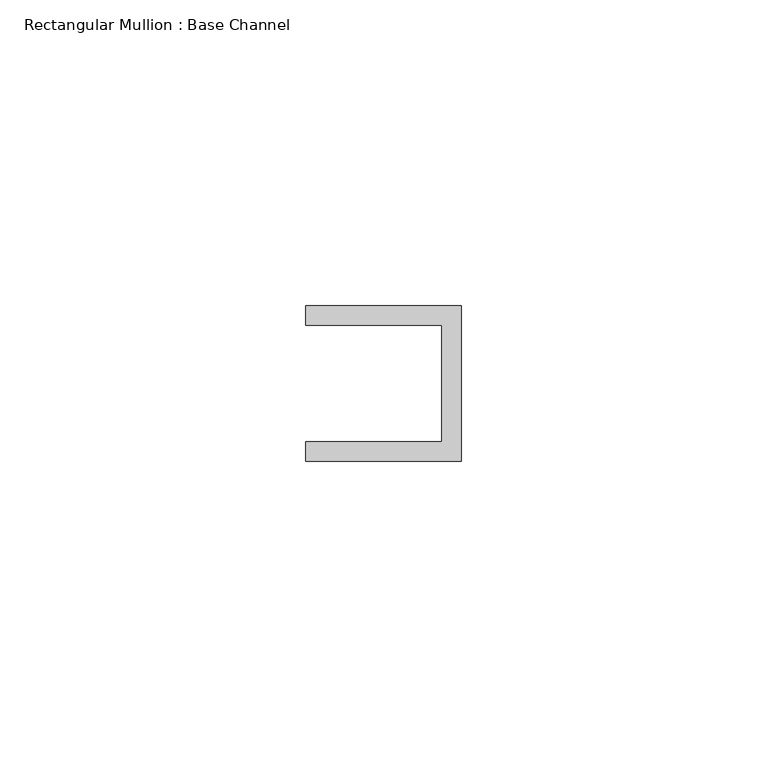
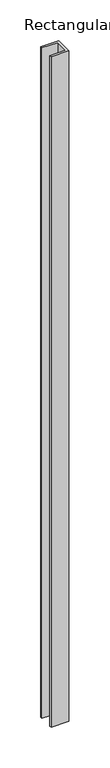
"""IFC4 building model written with IfcOpenShell, lengths in millimetres: member geometry, Rectangular Mullion : Base Channel."""

import ifcopenshell
import ifcopenshell.guid

model = None  # the IFC model being written
_history = None  # IfcOwnerHistory: only IFC2X3 demands one
_inside = {}  # id of a spatial element -> (the spatial element, [elements in it])
_under = {}  # id of a project, library or spatial element -> (it, [spatial elements below it])
_declared = {}  # id of a project -> (the project, [libraries it declares])
_typed = {}  # id of a type object -> (the type object, [elements of that type])
_made_of = {}  # id of a material, layer set ... -> (it, [elements and type objects made of it])


def new_model(schema):
    """Start an empty IFC model of exactly this schema.

    Asked for "IFC4X3", IfcOpenShell would pick the latest addendum, in which some entities
    have other attributes; the version numbers below select the first issue.
    IFC2X3 requires an IfcOwnerHistory on every rooted entity: one is made here for all.
    """
    global model, _history
    if schema == "IFC4X3":
        model = ifcopenshell.file(schema_version=(4, 3, 0, 0))
    else:
        model = ifcopenshell.file(schema=schema)
    _inside.clear()
    _under.clear()
    _declared.clear()
    _typed.clear()
    _made_of.clear()
    _history = None
    if model.schema == "IFC2X3":
        org = make("IfcOrganization", Name="unknown")
        user = make(
            "IfcPersonAndOrganization",
            ThePerson=make("IfcPerson", FamilyName="unknown"),
            TheOrganization=org,
        )
        app = make(
            "IfcApplication",
            ApplicationDeveloper=org,
            Version="unknown",
            ApplicationFullName="unknown",
            ApplicationIdentifier="unknown",
        )
        _history = make(
            "IfcOwnerHistory",
            OwningUser=user,
            OwningApplication=app,
            ChangeAction="ADDED",
            CreationDate=0,
        )
    return model


def make(cls, **values):
    """One entity of the class cls with the attributes given. An attribute that is None is left unset."""
    return model.create_entity(
        cls, **{name: value for name, value in values.items() if value is not None}
    )


def rooted(cls, **values):
    """An entity with a GlobalId (a new one), such as an element, a storey or a relation."""
    return make(cls, GlobalId=ifcopenshell.guid.new(), OwnerHistory=_history, **values)


def si_unit(unit_type, name, prefix=None):
    """IfcSIUnit, for example si_unit("LENGTHUNIT", "METRE", prefix="MILLI")."""
    return make("IfcSIUnit", UnitType=unit_type, Prefix=prefix, Name=name)


def assignment(units):
    """IfcUnitAssignment: the units of a project."""
    return None if units is None else make("IfcUnitAssignment", Units=units)


def point(xyz):
    """IfcCartesianPoint."""
    return None if xyz is None else make("IfcCartesianPoint", Coordinates=xyz)


def direction(xyz):
    """IfcDirection."""
    return None if xyz is None else make("IfcDirection", DirectionRatios=xyz)


def frame(location, z_axis=None, x_axis=None):
    """IfcAxis2Placement3D, a coordinate frame: its origin and axes. An axis left out is left unset."""
    return make(
        "IfcAxis2Placement3D",
        Location=point(location),
        Axis=direction(z_axis),
        RefDirection=direction(x_axis),
    )


def origin():
    """The frame at (0, 0, 0) with its axes left unset."""
    return frame((0.0, 0.0, 0.0))


def place(relative_to, where):
    """IfcLocalPlacement: puts the frame where relative to a parent placement (None: the world)."""
    return make(
        "IfcLocalPlacement", PlacementRelTo=relative_to, RelativePlacement=where
    )


def context(
    kind, dimensions, precision=None, world=None, true_north=None, identifier=None
):
    """IfcGeometricRepresentationContext, for example the 3D "Model" context."""
    return make(
        "IfcGeometricRepresentationContext",
        ContextIdentifier=identifier,
        ContextType=kind,
        CoordinateSpaceDimension=dimensions,
        Precision=precision,
        WorldCoordinateSystem=world,
        TrueNorth=true_north,
    )


def project(units=None, contexts=None):
    """IfcProject with its units and contexts."""
    return rooted(
        "IfcProject",
        Name="project",
        RepresentationContexts=contexts,
        UnitsInContext=assignment(units),
    )


def spatial(cls, under=None, at=None, **own):
    """A site, building, storey or space (cls), placed at a placement, below another one or the project."""
    s = rooted(cls, ObjectPlacement=at, **own)
    if under is not None:
        _under.setdefault(under.id(), (under, []))[1].append(s)
    return s


def polyline(points):
    """IfcPolyline through the points."""
    return make("IfcPolyline", Points=[point(p) for p in points])


def outline(outer, holes=None, kind="AREA"):
    """IfcArbitraryClosedProfileDef: a profile drawn as a closed curve; with holes, ...WithVoids."""
    if holes is None:
        return make("IfcArbitraryClosedProfileDef", ProfileType=kind, OuterCurve=outer)
    return make(
        "IfcArbitraryProfileDefWithVoids",
        ProfileType=kind,
        OuterCurve=outer,
        InnerCurves=holes,
    )


def extrude(swept, where, along, depth):
    """IfcExtrudedAreaSolid: the profile swept, set in the frame where, extruded along a direction by depth."""
    return make(
        "IfcExtrudedAreaSolid",
        SweptArea=swept,
        Position=where,
        ExtrudedDirection=direction(along),
        Depth=depth,
    )


def shape(context_of_items, identifier, shape_type, items):
    """IfcShapeRepresentation: the items that make up one representation, for example the "Body"."""
    return make(
        "IfcShapeRepresentation",
        ContextOfItems=context_of_items,
        RepresentationIdentifier=identifier,
        RepresentationType=shape_type,
        Items=items,
    )


def source(mapping_origin, context_of_items, identifier, shape_type, items):
    """IfcRepresentationMap: a shape defined once, which mapped items show again and again."""
    return make(
        "IfcRepresentationMap",
        MappingOrigin=mapping_origin,
        MappedRepresentation=shape(context_of_items, identifier, shape_type, items),
    )


def transform(
    local_origin,
    x_axis=None,
    y_axis=None,
    z_axis=None,
    scale=None,
    scale2=None,
    scale3=None,
    uniform=True,
):
    """IfcCartesianTransformationOperator3D, or its non-uniform kind. x_axis, y_axis, z_axis: its Axis1, 2, 3."""
    if uniform:
        return make(
            "IfcCartesianTransformationOperator3D",
            Axis1=direction(x_axis),
            Axis2=direction(y_axis),
            LocalOrigin=point(local_origin),
            Scale=scale,
            Axis3=direction(z_axis),
        )
    return make(
        "IfcCartesianTransformationOperator3DnonUniform",
        Axis1=direction(x_axis),
        Axis2=direction(y_axis),
        LocalOrigin=point(local_origin),
        Scale=scale,
        Axis3=direction(z_axis),
        Scale2=scale2,
        Scale3=scale3,
    )


def mapped(mapping_source, mapping_target):
    """IfcMappedItem: shows the shape of a source again, moved by a transform."""
    return make(
        "IfcMappedItem", MappingSource=mapping_source, MappingTarget=mapping_target
    )


def made_of(thing, what):
    """Note that an element or type object is made of a material, layer set ...; save() writes the relation."""
    if what is not None:
        _made_of.setdefault(what.id(), (what, []))[1].append(thing)
    return thing


def element(
    cls,
    number,
    at=None,
    inside=None,
    cuts=None,
    type_object=None,
    material=None,
    context=None,
    identifier="Body",
    shape_type=None,
    held_by="IfcProductDefinitionShape",
    body=None,
    shapes=None,
    **own,
):
    """One element of the class cls, such as IfcWall. Its Tag is "e" and its number.

    at: its placement. inside: the storey or other place that contains it. cuts: it is an
    opening in that element (IfcRelVoidsElement). A single representation is given by context,
    identifier, shape_type and body (its items); several are given by shapes. held_by: the class
    of the entity that holds the representations. save() writes the other relations.
    """
    e = rooted(cls, Tag="e%d" % number, ObjectPlacement=at, **own)
    if body is not None:
        shapes = [shape(context, identifier, shape_type, body)]
    if shapes is not None:
        e.Representation = make(held_by, Representations=shapes)
    if inside is not None:
        _inside.setdefault(inside.id(), (inside, []))[1].append(e)
    if cuts is not None:
        rooted(
            "IfcRelVoidsElement", RelatingBuildingElement=cuts, RelatedOpeningElement=e
        )
    if type_object is not None:
        _typed.setdefault(type_object.id(), (type_object, []))[1].append(e)
    return made_of(e, material)


def aggregate(whole, parts):
    """IfcRelAggregates: a whole, such as a stair, and the parts it consists of."""
    return rooted("IfcRelAggregates", RelatingObject=whole, RelatedObjects=parts)


def save(model, path):
    """Write the relations noted so far, then the file.

    IfcRelAggregates (storeys below a building ...), IfcRelContainedInSpatialStructure (elements
    in a storey), IfcRelDefinesByType, IfcRelAssociatesMaterial and IfcRelDeclares: one each for
    every whole, place, type object, material and project.
    """
    for whole, parts in _under.values():
        aggregate(whole, parts)
    for where, things in _inside.values():
        rooted(
            "IfcRelContainedInSpatialStructure",
            RelatedElements=things,
            RelatingStructure=where,
        )
    for kind, things in _typed.values():
        rooted("IfcRelDefinesByType", RelatedObjects=things, RelatingType=kind)
    for what, things in _made_of.values():
        rooted("IfcRelAssociatesMaterial", RelatedObjects=things, RelatingMaterial=what)
    for by, libraries in _declared.values():
        rooted("IfcRelDeclares", RelatingContext=by, RelatedDefinitions=libraries)
    model.write(path)


def rectangular_mullion_base_channel_45555192(model_context):
    return source(origin(), model_context, "Body", "SweptSolid", [
        extrude(outline(polyline([(0.0, -12.7), (-25.4, -12.7), (-25.4, -9.525), (-3.175, -9.525), (-3.175, 9.525), (-25.4, 9.525), (-25.4, 12.7), (0.0, 12.7), (0.0, -12.7)])), frame((0.0, 0.0, -1005.4166667), z_axis=(0.0, 0.0, 1.0), x_axis=(1.0, 0.0, 0.0)), (0.0, 0.0, 1.0), 1005.4166667),
    ])


if __name__ == "__main__":
    model = new_model("IFC4")
    model_context = context("Model", 3, world=origin())
    ifc_project = project(units=[si_unit("LENGTHUNIT", "METRE", prefix="MILLI")], contexts=[model_context])
    site = spatial("IfcSite", under=ifc_project)
    building = spatial("IfcBuilding", under=site)
    placement = place(None, origin())
    rectangular_mullion_base_channel_shape = rectangular_mullion_base_channel_45555192(model_context)
    element("IfcMember", 1, ObjectType="Rectangular Mullion : Base Channel", at=placement, inside=building, context=model_context, shape_type="MappedRepresentation", body=[
        mapped(rectangular_mullion_base_channel_shape, transform((0.0, 0.0, 0.0), x_axis=(1.0, 0.0, 0.0), y_axis=(0.0, 1.0, 0.0), z_axis=(0.0, 0.0, 1.0))),
    ])
    save(model, "model.ifc")

# Revit data of these elements
# Type "Rectangular Mullion : Base Channel"
#   built-in parameter 1007322 = 0.0833333 (stored number, unit not read)
#   built-in parameter 1007321 = 0.0416667 (stored number, unit not read)
#   built-in parameter 1007320 = -0.03125 (stored number, unit not read)
# Element 1 (IfcMember, "Rectangular Mullion : Base Channel")
#   Materials on its faces: "ALUM"
# Materials
#   "ALUM": class "Generic", colour RGB 157 157 157, transparency 0, Cost = 0
